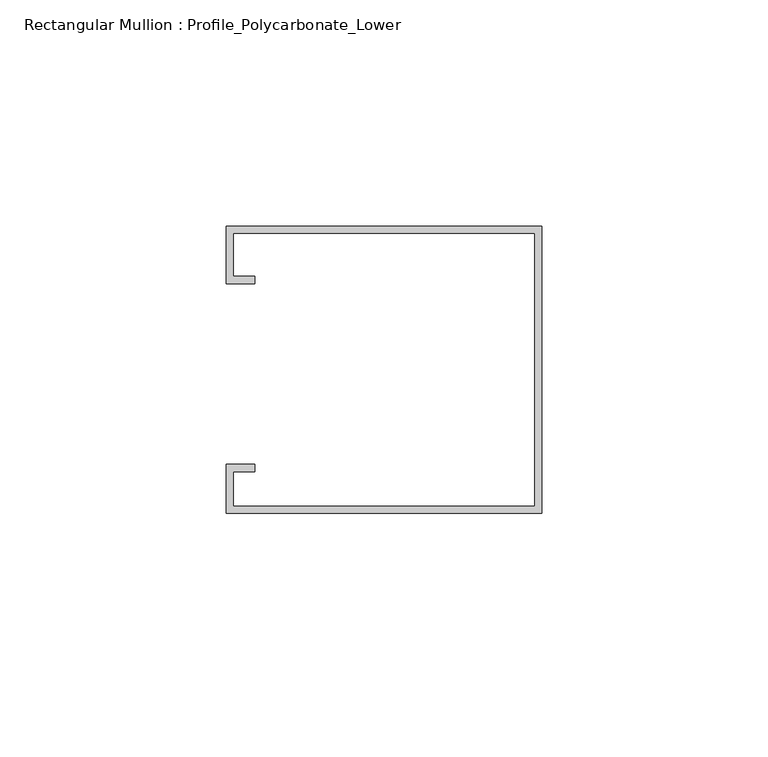
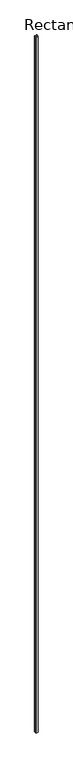
"""IFC4 building model written with IfcOpenShell, lengths in millimetres: member geometry, Rectangular Mullion : Profile_Polycarbonate_Lower."""

from ifc_helpers import new_model, si_unit, frame, origin, place, context, project, spatial, polyline, outline, extrude, source, transform, mapped, element, save


def rectangular_mullion_profile_polycarbonate_lower_fe6fa02e(model_context):
    return source(origin(), model_context, "Body", "SweptSolid", [
        extrude(outline(polyline([(0.0, 32.7), (0.0, -30.8), (-69.85, -30.8), (-69.85, -20.0), (-63.5, -20.0), (-63.5, -21.5875), (-68.2625, -21.5875), (-68.2625, -29.2125), (-1.5875, -29.2125), (-1.5875, 31.1125), (-68.2625, 31.1125), (-68.2625, 21.5875), (-63.5, 21.5875), (-63.5, 20.0), (-69.85, 20.0), (-69.85, 32.7), (0.0, 32.7)])), frame((0.0, 0.0, -21972.5875), z_axis=(0.0, 0.0, 1.0), x_axis=(1.0, 0.0, 0.0)), (0.0, 0.0, 1.0), 21972.5875),
    ])


if __name__ == "__main__":
    model = new_model("IFC4")
    model_context = context("Model", 3, world=origin())
    ifc_project = project(units=[si_unit("LENGTHUNIT", "METRE", prefix="MILLI")], contexts=[model_context])
    site = spatial("IfcSite", under=ifc_project)
    building = spatial("IfcBuilding", under=site)
    placement = place(None, origin())
    rectangular_mullion_profile_polycarbonate_lower_shape = rectangular_mullion_profile_polycarbonate_lower_fe6fa02e(model_context)
    element("IfcMember", 1, ObjectType="Rectangular Mullion : Profile_Polycarbonate_Lower", at=placement, inside=building, context=model_context, shape_type="MappedRepresentation", body=[
        mapped(rectangular_mullion_profile_polycarbonate_lower_shape, transform((0.0, 0.0, 0.0), x_axis=(1.0, 0.0, 0.0), y_axis=(0.0, 1.0, 0.0), z_axis=(0.0, 0.0, 1.0))),
    ])
    save(model, "model.ifc")

# Revit data of these elements
# Type "Rectangular Mullion : Profile_Polycarbonate_Lower"
#   built-in parameter 1007322 = 0.208333 (stored number, unit not read)
#   built-in parameter 1007321 = 0 (stored number, unit not read)
#   built-in parameter 1007320 = 0.00520833 (stored number, unit not read)
# Element 1 (IfcMember, "Rectangular Mullion : Profile_Polycarbonate_Lower")
#   Materials on its faces: "ALUMINUM PROFILE AT POLYCARBONATE PANEL"
# Materials
#   "ALUMINUM PROFILE AT POLYCARBONATE PANEL": class "Metal", colour RGB 244 244 244, transparency 0, Description = "Aluminum 6061", Cost = 0
